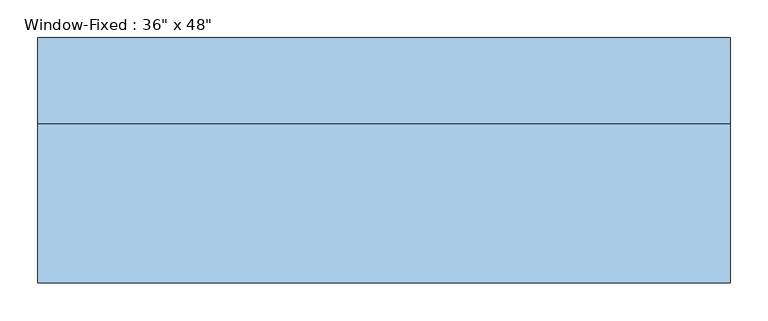
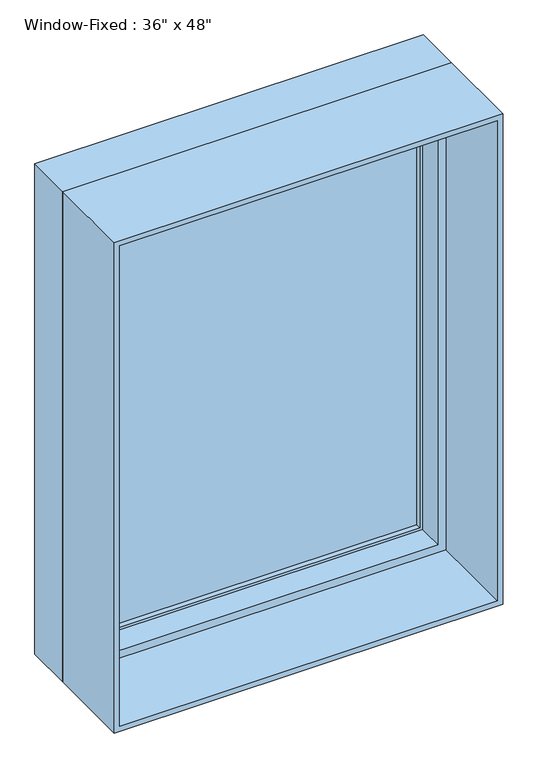
"""IFC4 building model written with IfcOpenShell, lengths in millimetres: window geometry."""

from ifc_helpers import new_model, si_unit, frame, origin, place, context, project, spatial, polyline, outline, extrude, faceted_brep, source, transform, mapped, element, save


def window_751a074a(model_context):
    return source(origin(), model_context, "Body", "SolidModel", [
        extrude(outline(polyline([(419.1, 152.4), (419.1, 146.05), (-419.1, 146.05), (-419.1, 152.4), (419.1, 152.4)])), frame((0.0, 0.0, 952.5), z_axis=(0.0, 0.0, 1.0), x_axis=(1.0, 0.0, 0.0)), (0.0, 0.0, 1.0), 1143.0),
        extrude(outline(polyline([(-419.1, 133.35), (-419.1, 139.7), (419.1, 139.7), (419.1, 133.35), (-419.1, 133.35)])), frame((0.0, 0.0, 952.5), z_axis=(0.0, 0.0, 1.0), x_axis=(1.0, 0.0, 0.0)), (0.0, 0.0, 1.0), 1143.0),
        extrude(outline(polyline([(927.1, 444.5), (2120.9, 444.5), (2120.9, -444.5), (927.1, -444.5), (927.1, 444.5)]), holes=[polyline([(952.5, -419.1), (2095.5, -419.1), (2095.5, 419.1), (952.5, 419.1), (952.5, -419.1)])]), frame((0.0, 120.65, 0.0), z_axis=(0.0, 1.0, 0.0), x_axis=(0.0, 0.0, 1.0)), (0.0, 0.0, 1.0), 44.45),
        extrude(outline(polyline([(2133.6, -457.2), (914.4, -457.2), (914.4, 457.2), (2133.6, 457.2), (2133.6, -457.2)]), holes=[polyline([(2120.9, 444.5), (927.1, 444.5), (927.1, -444.5), (2120.9, -444.5), (2120.9, 444.5)])]), frame((0.0, -152.4, 0.0), z_axis=(0.0, 1.0, 0.0), x_axis=(0.0, 0.0, 1.0)), (0.0, 0.0, 1.0), 209.55),
        faceted_brep([(457.2, 57.15, 2133.6), (457.2, 171.45, 2133.6), (-457.2, 171.45, 2133.6), (-457.2, 57.15, 2133.6), (-457.2, 171.45, 914.4), (-457.2, 57.15, 914.4), (457.2, 171.45, 914.4), (457.2, 57.15, 914.4), (425.45, 57.15, 2101.85), (425.45, 57.15, 946.15), (-425.45, 57.15, 946.15), (-425.45, 57.15, 2101.85), (-444.5, 171.45, 2120.9), (-444.5, 171.45, 927.1), (444.5, 171.45, 927.1), (444.5, 171.45, 2120.9), (425.45, 120.65, 2101.85), (-425.45, 120.65, 2101.85), (444.5, 120.65, 2120.9), (-444.5, 120.65, 2120.9), (-425.45, 120.65, 946.15), (-444.5, 120.65, 927.1), (425.45, 120.65, 946.15), (444.5, 120.65, 927.1)], [[[0, 1, 2, 3]], [[3, 2, 4, 5]], [[5, 4, 6, 7]], [[3, 5, 7, 0], [8, 9, 10, 11]], [[7, 6, 1, 0]], [[1, 6, 4, 2], [12, 13, 14, 15]], [[16, 8, 11, 17]], [[15, 18, 19, 12]], [[17, 11, 10, 20]], [[12, 19, 21, 13]], [[20, 10, 9, 22]], [[13, 21, 23, 14]], [[22, 9, 8, 16]], [[18, 23, 21, 19], [17, 20, 22, 16]], [[14, 23, 18, 15]]]),
    ])


if __name__ == "__main__":
    model = new_model("IFC4")
    model_context = context("Model", 3, world=origin())
    ifc_project = project(units=[si_unit("LENGTHUNIT", "METRE", prefix="MILLI")], contexts=[model_context])
    site = spatial("IfcSite", under=ifc_project)
    building = spatial("IfcBuilding", under=site)
    placement = place(None, origin())
    window_shape = window_751a074a(model_context)
    element("IfcWindow", 1, ObjectType="Window-Fixed : 36\" x 48\"", at=placement, inside=building, context=model_context, shape_type="MappedRepresentation", body=[
        mapped(window_shape, transform((0.0, 0.0, 0.0), x_axis=(1.0, 0.0, 0.0), y_axis=(0.0, 1.0, 0.0), z_axis=(0.0, 0.0, 1.0))),
    ])
    save(model, "model.ifc")

# Revit data of these elements
# Type "Window-Fixed : 36\" x 48\""
#   Type Mark = "H"
#   Fire Rating = "0.5h"
#   Assembly Code = "B2020100"
#   Analytic Construction = "Double glazing - domestic"
#   Window Inset [instance default] = 0' - 0"
#   Wall Thickness [instance default] = 0' - 6"
#   Visual Light Transmittance = 0.81
#   Thermal Resistance (R) = 1.8146 (h·ft²·°F)/BTU
#   Solar Heat Gain Coefficient = 0.76
#   Rough Width = 3' - 0 1/2"
#   Rough Height = 4' - 0 1/2"
#   Interior Wall Closure [instance default] = 0' - 2 1/4"
#   Height = 4' - 0"
#   Heat Transfer Coefficient (U) = 0.5511 BTU/(h·ft²·°F)
#   Frame Extension [instance default] = 0' - 0 1/4"
#   Exterior Wall Closure [instance default] = 0' - 1 1/4"
#   Extension Jamb [instance default] = 0' - 2 1/4"
#   Default Sill Height = 3' - 0"
#   Width = 3' - 0"
#   Muntin Visibility = yes
#   Interior Trim Visibility [instance default] = yes
#   Exterior Trim Visibility [instance default] = yes
#   Extension Jamb Visibility [instance default] = yes
#   Muntin Pattern = Muntin Pattern_2x2 : Muntin Pattern_2x2
#   Interior Trim Material = Wood - Stained
#   Interior Trim = Trim-Window-Interior-Flat : Picture Frame
#   Interior Frame Material = Wood - Stained
#   Glass Panel Material = Glass
#   Exterior Trim Material = Clad - White
#   Exterior Trim = Trim-Window-Exterior-Flat : with Sill
#   Exterior Frame Material = Clad - White
#   Wall Closure = (empty or 0)
# Element 1 (IfcWindow, "Window-Fixed : 36\" x 48\"")
#   Wall Thickness = 1' - 0"
#   Extension Jamb = 0' - 8 1/4"
#   Materials on its faces: "Wood - Stained", "Glass", "Clad - White"
# Materials
#   "Wood - Stained": class "Wood", colour RGB 224 178 126, transparency 0, Cost = 0
#   "Glass": class "Unassigned", colour RGB 0 128 192, transparency 0.75, Description = "Glass"
#   "Clad - White": class "Wood", colour RGB 242 242 238, transparency 0, Cost = 0
